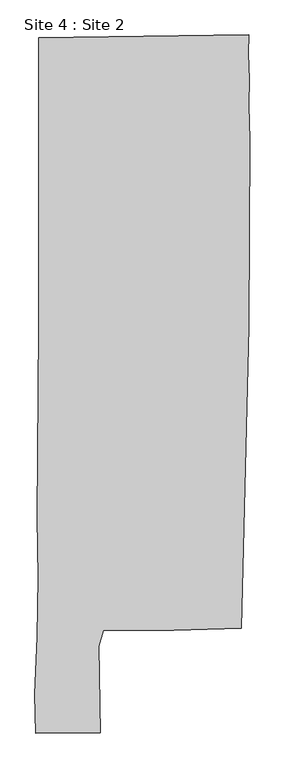
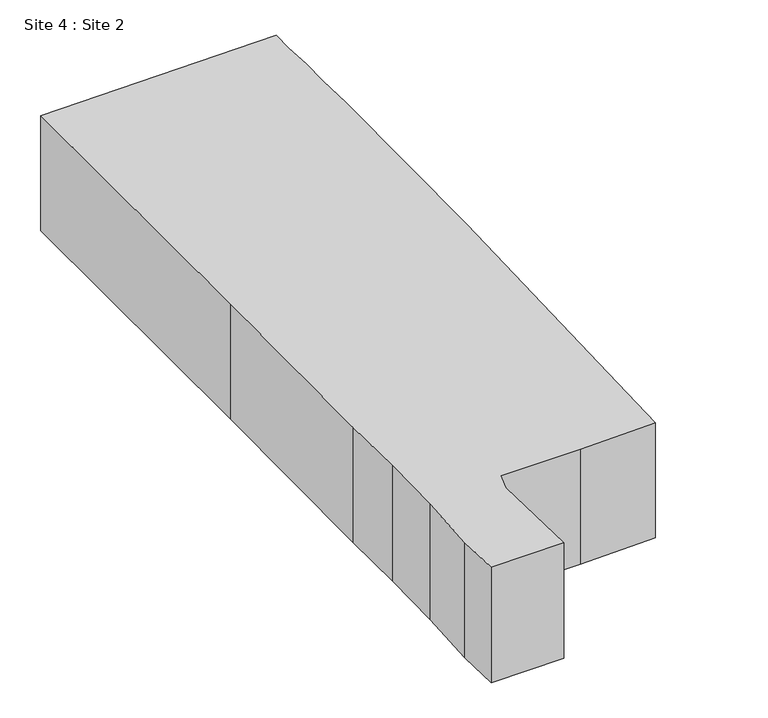
"""IFC4 building model written with IfcOpenShell, lengths in millimetres: geographic element geometry, Site 4 : Site 2."""

import ifcopenshell
import ifcopenshell.guid

model = None  # the IFC model being written
_history = None  # IfcOwnerHistory: only IFC2X3 demands one
_inside = {}  # id of a spatial element -> (the spatial element, [elements in it])
_under = {}  # id of a project, library or spatial element -> (it, [spatial elements below it])
_declared = {}  # id of a project -> (the project, [libraries it declares])
_typed = {}  # id of a type object -> (the type object, [elements of that type])
_made_of = {}  # id of a material, layer set ... -> (it, [elements and type objects made of it])


def new_model(schema):
    """Start an empty IFC model of exactly this schema.

    Asked for "IFC4X3", IfcOpenShell would pick the latest addendum, in which some entities
    have other attributes; the version numbers below select the first issue.
    IFC2X3 requires an IfcOwnerHistory on every rooted entity: one is made here for all.
    """
    global model, _history
    if schema == "IFC4X3":
        model = ifcopenshell.file(schema_version=(4, 3, 0, 0))
    else:
        model = ifcopenshell.file(schema=schema)
    _inside.clear()
    _under.clear()
    _declared.clear()
    _typed.clear()
    _made_of.clear()
    _history = None
    if model.schema == "IFC2X3":
        org = make("IfcOrganization", Name="unknown")
        user = make(
            "IfcPersonAndOrganization",
            ThePerson=make("IfcPerson", FamilyName="unknown"),
            TheOrganization=org,
        )
        app = make(
            "IfcApplication",
            ApplicationDeveloper=org,
            Version="unknown",
            ApplicationFullName="unknown",
            ApplicationIdentifier="unknown",
        )
        _history = make(
            "IfcOwnerHistory",
            OwningUser=user,
            OwningApplication=app,
            ChangeAction="ADDED",
            CreationDate=0,
        )
    return model


def make(cls, **values):
    """One entity of the class cls with the attributes given. An attribute that is None is left unset."""
    return model.create_entity(
        cls, **{name: value for name, value in values.items() if value is not None}
    )


def rooted(cls, **values):
    """An entity with a GlobalId (a new one), such as an element, a storey or a relation."""
    return make(cls, GlobalId=ifcopenshell.guid.new(), OwnerHistory=_history, **values)


def si_unit(unit_type, name, prefix=None):
    """IfcSIUnit, for example si_unit("LENGTHUNIT", "METRE", prefix="MILLI")."""
    return make("IfcSIUnit", UnitType=unit_type, Prefix=prefix, Name=name)


def assignment(units):
    """IfcUnitAssignment: the units of a project."""
    return None if units is None else make("IfcUnitAssignment", Units=units)


def point(xyz):
    """IfcCartesianPoint."""
    return None if xyz is None else make("IfcCartesianPoint", Coordinates=xyz)


def direction(xyz):
    """IfcDirection."""
    return None if xyz is None else make("IfcDirection", DirectionRatios=xyz)


def frame(location, z_axis=None, x_axis=None):
    """IfcAxis2Placement3D, a coordinate frame: its origin and axes. An axis left out is left unset."""
    return make(
        "IfcAxis2Placement3D",
        Location=point(location),
        Axis=direction(z_axis),
        RefDirection=direction(x_axis),
    )


def origin():
    """The frame at (0, 0, 0) with its axes left unset."""
    return frame((0.0, 0.0, 0.0))


def place(relative_to, where):
    """IfcLocalPlacement: puts the frame where relative to a parent placement (None: the world)."""
    return make(
        "IfcLocalPlacement", PlacementRelTo=relative_to, RelativePlacement=where
    )


def context(
    kind, dimensions, precision=None, world=None, true_north=None, identifier=None
):
    """IfcGeometricRepresentationContext, for example the 3D "Model" context."""
    return make(
        "IfcGeometricRepresentationContext",
        ContextIdentifier=identifier,
        ContextType=kind,
        CoordinateSpaceDimension=dimensions,
        Precision=precision,
        WorldCoordinateSystem=world,
        TrueNorth=true_north,
    )


def project(units=None, contexts=None):
    """IfcProject with its units and contexts."""
    return rooted(
        "IfcProject",
        Name="project",
        RepresentationContexts=contexts,
        UnitsInContext=assignment(units),
    )


def spatial(cls, under=None, at=None, **own):
    """A site, building, storey or space (cls), placed at a placement, below another one or the project."""
    s = rooted(cls, ObjectPlacement=at, **own)
    if under is not None:
        _under.setdefault(under.id(), (under, []))[1].append(s)
    return s


def polyline(points):
    """IfcPolyline through the points."""
    return make("IfcPolyline", Points=[point(p) for p in points])


def outline(outer, holes=None, kind="AREA"):
    """IfcArbitraryClosedProfileDef: a profile drawn as a closed curve; with holes, ...WithVoids."""
    if holes is None:
        return make("IfcArbitraryClosedProfileDef", ProfileType=kind, OuterCurve=outer)
    return make(
        "IfcArbitraryProfileDefWithVoids",
        ProfileType=kind,
        OuterCurve=outer,
        InnerCurves=holes,
    )


def extrude(swept, where, along, depth):
    """IfcExtrudedAreaSolid: the profile swept, set in the frame where, extruded along a direction by depth."""
    return make(
        "IfcExtrudedAreaSolid",
        SweptArea=swept,
        Position=where,
        ExtrudedDirection=direction(along),
        Depth=depth,
    )


def shape(context_of_items, identifier, shape_type, items):
    """IfcShapeRepresentation: the items that make up one representation, for example the "Body"."""
    return make(
        "IfcShapeRepresentation",
        ContextOfItems=context_of_items,
        RepresentationIdentifier=identifier,
        RepresentationType=shape_type,
        Items=items,
    )


def source(mapping_origin, context_of_items, identifier, shape_type, items):
    """IfcRepresentationMap: a shape defined once, which mapped items show again and again."""
    return make(
        "IfcRepresentationMap",
        MappingOrigin=mapping_origin,
        MappedRepresentation=shape(context_of_items, identifier, shape_type, items),
    )


def transform(
    local_origin,
    x_axis=None,
    y_axis=None,
    z_axis=None,
    scale=None,
    scale2=None,
    scale3=None,
    uniform=True,
):
    """IfcCartesianTransformationOperator3D, or its non-uniform kind. x_axis, y_axis, z_axis: its Axis1, 2, 3."""
    if uniform:
        return make(
            "IfcCartesianTransformationOperator3D",
            Axis1=direction(x_axis),
            Axis2=direction(y_axis),
            LocalOrigin=point(local_origin),
            Scale=scale,
            Axis3=direction(z_axis),
        )
    return make(
        "IfcCartesianTransformationOperator3DnonUniform",
        Axis1=direction(x_axis),
        Axis2=direction(y_axis),
        LocalOrigin=point(local_origin),
        Scale=scale,
        Axis3=direction(z_axis),
        Scale2=scale2,
        Scale3=scale3,
    )


def mapped(mapping_source, mapping_target):
    """IfcMappedItem: shows the shape of a source again, moved by a transform."""
    return make(
        "IfcMappedItem", MappingSource=mapping_source, MappingTarget=mapping_target
    )


def made_of(thing, what):
    """Note that an element or type object is made of a material, layer set ...; save() writes the relation."""
    if what is not None:
        _made_of.setdefault(what.id(), (what, []))[1].append(thing)
    return thing


def element(
    cls,
    number,
    at=None,
    inside=None,
    cuts=None,
    type_object=None,
    material=None,
    context=None,
    identifier="Body",
    shape_type=None,
    held_by="IfcProductDefinitionShape",
    body=None,
    shapes=None,
    **own,
):
    """One element of the class cls, such as IfcWall. Its Tag is "e" and its number.

    at: its placement. inside: the storey or other place that contains it. cuts: it is an
    opening in that element (IfcRelVoidsElement). A single representation is given by context,
    identifier, shape_type and body (its items); several are given by shapes. held_by: the class
    of the entity that holds the representations. save() writes the other relations.
    """
    e = rooted(cls, Tag="e%d" % number, ObjectPlacement=at, **own)
    if body is not None:
        shapes = [shape(context, identifier, shape_type, body)]
    if shapes is not None:
        e.Representation = make(held_by, Representations=shapes)
    if inside is not None:
        _inside.setdefault(inside.id(), (inside, []))[1].append(e)
    if cuts is not None:
        rooted(
            "IfcRelVoidsElement", RelatingBuildingElement=cuts, RelatedOpeningElement=e
        )
    if type_object is not None:
        _typed.setdefault(type_object.id(), (type_object, []))[1].append(e)
    return made_of(e, material)


def aggregate(whole, parts):
    """IfcRelAggregates: a whole, such as a stair, and the parts it consists of."""
    return rooted("IfcRelAggregates", RelatingObject=whole, RelatedObjects=parts)


def save(model, path):
    """Write the relations noted so far, then the file.

    IfcRelAggregates (storeys below a building ...), IfcRelContainedInSpatialStructure (elements
    in a storey), IfcRelDefinesByType, IfcRelAssociatesMaterial and IfcRelDeclares: one each for
    every whole, place, type object, material and project.
    """
    for whole, parts in _under.values():
        aggregate(whole, parts)
    for where, things in _inside.values():
        rooted(
            "IfcRelContainedInSpatialStructure",
            RelatedElements=things,
            RelatingStructure=where,
        )
    for kind, things in _typed.values():
        rooted("IfcRelDefinesByType", RelatedObjects=things, RelatingType=kind)
    for what, things in _made_of.values():
        rooted("IfcRelAssociatesMaterial", RelatedObjects=things, RelatingMaterial=what)
    for by, libraries in _declared.values():
        rooted("IfcRelDeclares", RelatingContext=by, RelatedDefinitions=libraries)
    model.write(path)


def site_4_site_2_d3c7b1b5(model_context):
    return source(origin(), model_context, "Body", "SweptSolid", [
        extrude(outline(polyline([(47069.739469, 118051.0435782), (47043.2485504, 116222.4753159), (47109.5144512, 113782.9125819), (47019.7812823, 100575.0298085), (46507.5402416, 79244.5499285), (41729.8960793, 79110.547942), (36750.5493833, 79081.0765167), (36429.590646, 77968.03341), (36544.4654549, 71869.8200444), (31971.4757273, 71834.4616257), (31909.6213599, 74578.828126), (32070.0814264, 78640.8413742), (32130.4224653, 82805.9558551), (32090.6432502, 87074.0869127), (32183.3240873, 100485.1438761), (32175.8424465, 121010.2431952), (47013.7719724, 121201.7585813), (46994.6390291, 119881.0836194), (47069.739469, 118051.0435782)])), frame((0.0, 0.0, 266395.2), z_axis=(0.0, 0.0, 1.0), x_axis=(1.0, 0.0, 0.0)), (0.0, 0.0, 1.0), 7620.0),
    ])


if __name__ == "__main__":
    model = new_model("IFC4")
    model_context = context("Model", 3, world=origin())
    ifc_project = project(units=[si_unit("LENGTHUNIT", "METRE", prefix="MILLI")], contexts=[model_context])
    site = spatial("IfcSite", under=ifc_project)
    building = spatial("IfcBuilding", under=site)
    placement = place(None, origin())
    site_4_site_2_shape = site_4_site_2_d3c7b1b5(model_context)
    element("IfcGeographicElement", 1, ObjectType="Site 4 : Site 2", at=placement, inside=building, context=model_context, shape_type="MappedRepresentation", body=[
        mapped(site_4_site_2_shape, transform((0.0, 0.0, 0.0), x_axis=(1.0, 0.0, 0.0), y_axis=(0.0, 1.0, 0.0), z_axis=(0.0, 0.0, 1.0))),
    ])
    save(model, "model.ifc")

# Revit data of these elements
# Element 1 (IfcGeographicElement, "Site 4 : Site 2")
#   Materials on its faces: "EXISTING BUILDING"
# Materials
#   "EXISTING BUILDING": class "Generic", colour RGB 120 120 120, transparency 0, Cost = 0
